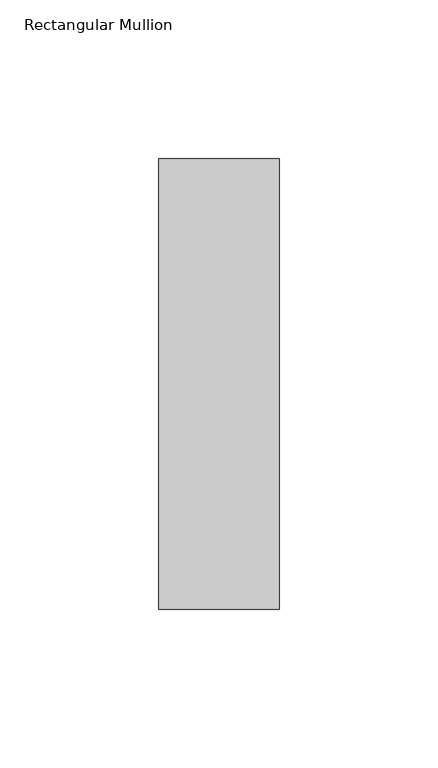
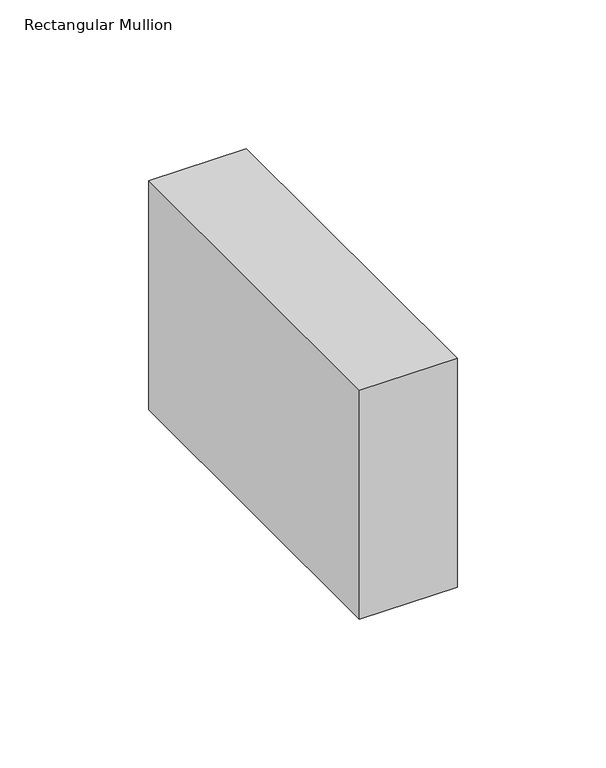
"""IFC4 building model written with IfcOpenShell, lengths in millimetres: member geometry, Rectangular Mullion : NLRS_21_CWM_hsb-regel 38x142_gen_rsf."""

from ifc_helpers import new_model, si_unit, frame, origin, place, context, project, spatial, polyline, outline, extrude, source, transform, mapped, element, save


def rectangular_mullion_b209e97a(model_context):
    return source(origin(), model_context, "Body", "SweptSolid", [
        extrude(outline(polyline([(-38.0, -71.0), (-38.0, 71.0), (0.0, 71.0), (0.0, -71.0), (-38.0, -71.0)])), frame((0.0, 0.0, -94.1558939), z_axis=(0.0, 0.0, 1.0), x_axis=(1.0, 0.0, 0.0)), (0.0, 0.0, 1.0), 94.1558939),
    ])


if __name__ == "__main__":
    model = new_model("IFC4")
    model_context = context("Model", 3, world=origin())
    ifc_project = project(units=[si_unit("LENGTHUNIT", "METRE", prefix="MILLI")], contexts=[model_context])
    site = spatial("IfcSite", under=ifc_project)
    building = spatial("IfcBuilding", under=site)
    placement = place(None, origin())
    rectangular_mullion_shape = rectangular_mullion_b209e97a(model_context)
    element("IfcMember", 1, ObjectType="Rectangular Mullion : NLRS_21_CWM_hsb-regel 38x142_gen_rsf", at=placement, inside=building, context=model_context, shape_type="MappedRepresentation", body=[
        mapped(rectangular_mullion_shape, transform((0.0, 0.0, 0.0), x_axis=(1.0, 0.0, 0.0), y_axis=(0.0, 1.0, 0.0), z_axis=(0.0, 0.0, 1.0))),
    ])
    save(model, "model.ifc")

# Revit data of these elements
# Type "Rectangular Mullion : NLRS_21_CWM_hsb-regel 38x142_gen_rsf"
#   Export Type to IFC As = "IfcWall"
#   Type IfcGUID = "07M7mRoiH1CR8m_RSKIwpF"
#   Assembly Code = "21.10"
#   built-in parameter 1007322 = 0.465879 (stored number, unit not read)
#   built-in parameter 1007321 = 0.062336 (stored number, unit not read)
#   built-in parameter 1007320 = 0.062336 (stored number, unit not read)
# Element 1 (IfcMember, "Rectangular Mullion : NLRS_21_CWM_hsb-regel 38x142_gen_rsf")
#   Materials on its faces: "NLRS_i2_hout naaldhout vuren_gen_rsf"
# Materials
#   "NLRS_i2_hout naaldhout vuren_gen_rsf": class "I - Hout", colour RGB 234 199 147, transparency 0, Keynote = "i2", Manufacturer = "Revit Standards Foundation", URL = "www.revitstandards.org", Description = "hout vuren", Cost = 0
